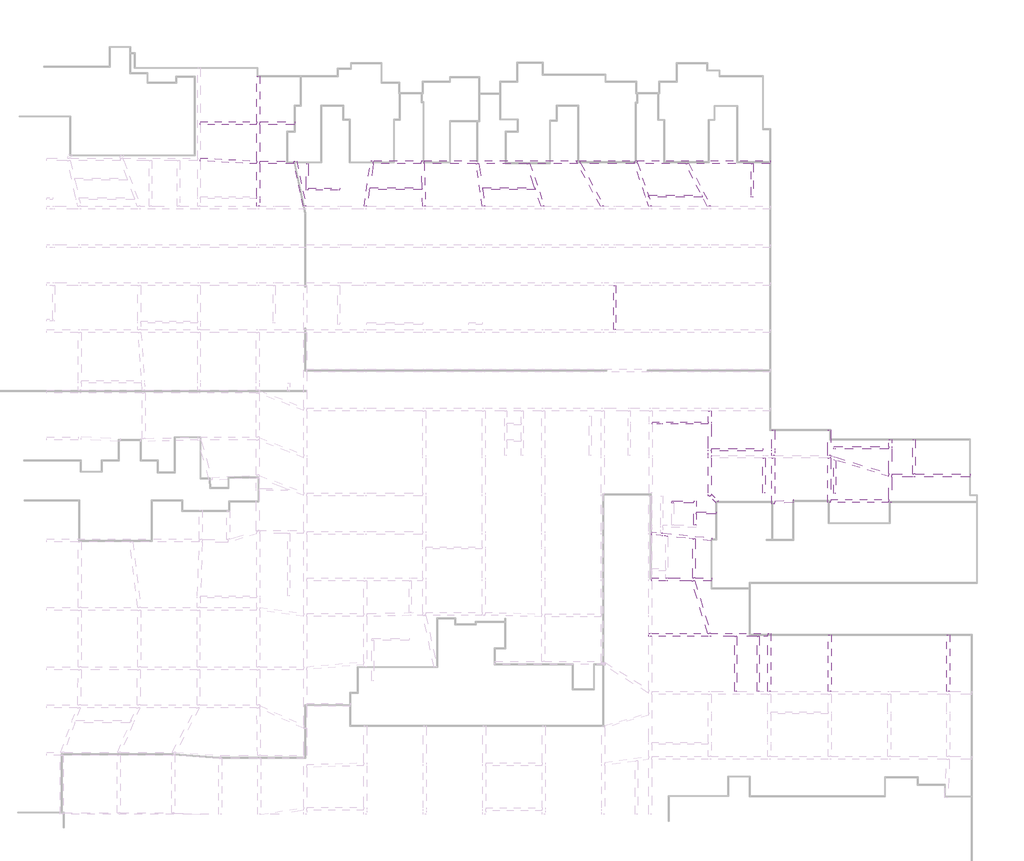
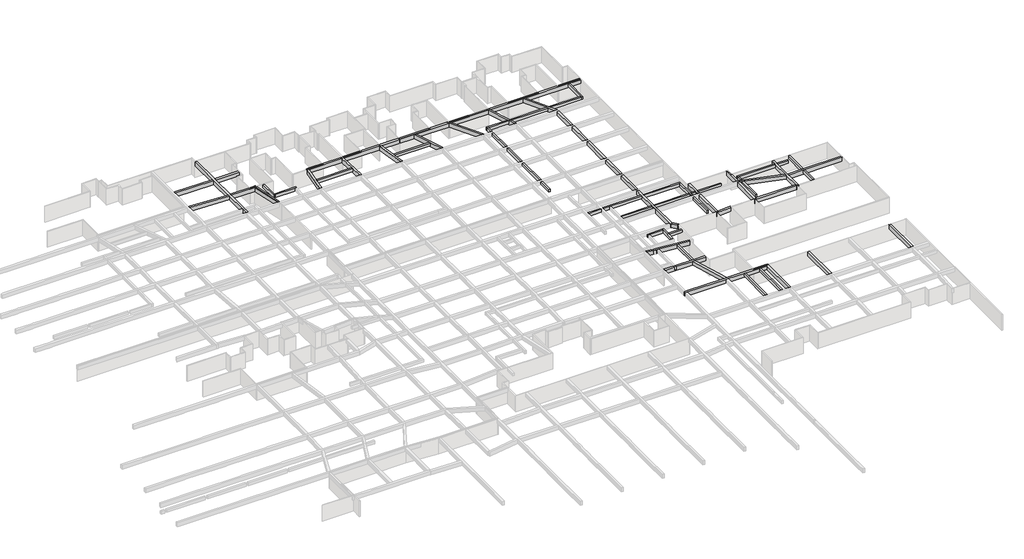
# One storey, part 16 of 16: 54 beams.
"""IFC4 building model written with IfcOpenShell, lengths in millimetres."""

from ifc_helpers import new_model, si_unit, frame, origin, place, context, project, spatial, polyline, outline, extrude, faceted_brep, element, save

model = new_model("IFC4")

# Units and contexts
model_context = context("Model", 3, world=origin())
ifc_project = project(units=[si_unit("LENGTHUNIT", "METRE", prefix="MILLI")], contexts=[model_context])

# Site, building, storey
site = spatial("IfcSite", under=ifc_project)
building = spatial("IfcBuilding", under=site)
storey = spatial("IfcBuildingStorey", under=building, Name="户型图", Elevation=0.0)

# Beams
placement = place(None, origin())
element("IfcBeam", 1, ObjectType="混凝土 - 矩形梁 : KL_beam", at=placement, inside=storey, context=model_context, shape_type="Brep", body=[
    faceted_brep([(134874.2374796, 207962.1094056, 3300.0), (135274.2374796, 207962.1094056, 3300.0), (135274.2374796, 207962.1094056, 2500.0), (134874.2374796, 207962.1094056, 2500.0), (134874.2374796, 201812.9009701, 3300.0), (134874.2374796, 201412.9009701, 3300.0), (134874.2374796, 196462.0408085, 3300.0), (134874.2374796, 196061.4918701, 3300.0), (134874.2374796, 191637.5884701, 3300.0), (134874.2374796, 191337.5884701, 3300.0), (134874.2374796, 190295.7397162, 3300.0), (135274.2374796, 190295.7397162, 3300.0), (135274.2374796, 191337.5884701, 3300.0), (135274.2374796, 191637.5884701, 3300.0), (135274.2374796, 196067.301294, 3300.0), (135274.2374796, 196467.301294, 3300.0), (135274.2374796, 201412.9009701, 3300.0), (135274.2374796, 201812.9009701, 3300.0), (135274.2374796, 190295.7397162, 2500.0), (135274.2374796, 196067.301294, 2500.0), (135274.2374796, 196467.301294, 2500.0), (135274.2374796, 201412.9009701, 2500.0), (135274.2374796, 201812.9009701, 2500.0), (134874.2374796, 190295.7397162, 2500.0), (134874.2374796, 196061.4918701, 2500.0), (134874.2374796, 196462.0408085, 2500.0), (134874.2374796, 201412.9009701, 2500.0), (134874.2374796, 201812.9009701, 2500.0)], [[[0, 1, 2, 3]], [[1, 0, 4, 5, 6, 7, 8, 9, 10, 11, 12, 13, 14, 15, 16, 17]], [[2, 1, 17, 16, 15, 14, 13, 12, 11, 18, 19, 20, 21, 22]], [[3, 2, 22, 21, 20, 19, 18, 23, 24, 25, 26, 27]], [[0, 3, 27, 26, 25, 24, 23, 10, 9, 8, 7, 6, 5, 4]], [[11, 10, 23, 18]]]),
])
element("IfcBeam", 2, ObjectType="混凝土 - 矩形梁 : KL_beam", at=placement, inside=storey, context=model_context, shape_type="SweptSolid", body=[
    extrude(outline(polyline([(127216.2109037, 196462.8320366), (127216.2109037, 196863.380975), (134874.2374796, 196462.0408085), (134874.2374796, 196061.4918701), (127216.2109037, 196462.8320366)])), frame((0.0, 0.0, 2500.0), z_axis=(0.0, 0.0, 1.0), x_axis=(1.0, 0.0, 0.0)), (0.0, 0.0, 1.0), 800.0),
])
element("IfcBeam", 3, ObjectType="混凝土 - 矩形梁 : KL_beam", at=placement, inside=storey, context=model_context, shape_type="SweptSolid", body=[
    extrude(outline(polyline([(127216.2109037, 201412.9009701), (127216.2109037, 201812.9009701), (134874.2374796, 201812.9009701), (134874.2374796, 201412.9009701), (127216.2109037, 201412.9009701)])), frame((0.0, 0.0, 2500.0), z_axis=(0.0, 0.0, 1.0), x_axis=(1.0, 0.0, 0.0)), (0.0, 0.0, 1.0), 800.0),
])
element("IfcBeam", 4, ObjectType="混凝土 - 矩形梁 : KL_beam", at=placement, inside=storey, context=model_context, shape_type="Brep", body=[
    faceted_brep([(196626.5590225, 189895.7397162, 3300.0), (196226.5590225, 189895.7397162, 3300.0), (196226.5590225, 185072.5884701, 3300.0), (196626.5590225, 185072.5884701, 3300.0), (196226.5590225, 189895.7397162, 2500.0), (196226.5590225, 185072.5884701, 2500.0), (196626.5590225, 189895.7397162, 2500.0), (196626.5590225, 185072.5884701, 2500.0)], [[[0, 1, 2, 3]], [[1, 4, 5, 2]], [[4, 6, 7, 5]], [[6, 0, 3, 7]], [[1, 0, 6, 4]], [[3, 2, 5, 7]]]),
    faceted_brep([(196226.5590225, 184672.5884701, 3300.0), (196626.5590225, 184672.5884701, 3300.0), (196626.5590225, 184672.5884701, 2500.0), (196226.5590225, 184672.5884701, 2500.0), (196626.5590225, 179912.5884701, 3300.0), (196226.5590225, 179912.5884701, 3300.0), (196226.5590225, 179912.5884701, 2500.0), (196626.5590225, 179912.5884701, 2500.0)], [[[0, 1, 2, 3]], [[4, 5, 6, 7]], [[1, 0, 5, 4]], [[0, 3, 6, 5]], [[3, 2, 7, 6]], [[2, 1, 4, 7]]]),
    faceted_brep([(196626.5590225, 179512.5884701, 3300.0), (196226.5590225, 179512.5884701, 3300.0), (196226.5590225, 173512.5884701, 3300.0), (196626.5590225, 173512.5884701, 3300.0), (196226.5590225, 179512.5884701, 2500.0), (196226.5590225, 173512.5884701, 2500.0), (196626.5590225, 179512.5884701, 2500.0), (196626.5590225, 173512.5884701, 2500.0)], [[[0, 1, 2, 3]], [[1, 4, 5, 2]], [[4, 6, 7, 5]], [[6, 0, 3, 7]], [[1, 0, 6, 4]], [[3, 2, 5, 7]]]),
    faceted_brep([(196226.5590225, 173112.5884701, 3300.0), (196626.5590225, 173112.5884701, 3300.0), (196626.5590225, 173112.5884701, 2500.0), (196226.5590225, 173112.5884701, 2500.0), (196626.5590225, 168162.578939, 3300.0), (196226.5590225, 168162.578939, 3300.0), (196226.5590225, 168162.578939, 2500.0), (196626.5590225, 168162.578939, 2500.0)], [[[0, 1, 2, 3]], [[4, 5, 6, 7]], [[1, 0, 5, 4]], [[0, 3, 6, 5]], [[3, 2, 7, 6]], [[2, 1, 4, 7]]]),
    faceted_brep([(196226.5590225, 162447.0169772, 3300.0), (196626.5590225, 162447.0169772, 3300.0), (196626.5590225, 162447.0169772, 2500.0), (196226.5590225, 162447.0169772, 2500.0), (196626.5590225, 150902.424794, 3300.0), (196343.71631, 150902.424794, 3300.0), (196226.5590225, 150902.424794, 3300.0), (196226.5590225, 150902.424794, 2500.0), (196343.71631, 150902.424794, 2500.0), (196626.5590225, 150902.424794, 2500.0), (196626.5590225, 151185.2675065, 3300.0), (196626.5590225, 156044.0267812, 3300.0), (196626.5590225, 156444.0267812, 3300.0), (196626.5590225, 157037.5884701, 3300.0), (196626.5590225, 157337.5884701, 3300.0), (196626.5590225, 160683.8998965, 3300.0), (196626.5590225, 160983.8998965, 3300.0), (196226.5590225, 160983.8998965, 3300.0), (196226.5590225, 160683.8998965, 3300.0), (196226.5590225, 157337.5884701, 3300.0), (196226.5590225, 157037.5884701, 3300.0), (196226.5590225, 156444.0267812, 3300.0), (196226.5590225, 156044.0267812, 3300.0), (196226.5590225, 151302.424794, 3300.0), (196226.5590225, 156444.0267812, 2500.0), (196226.5590225, 156044.0267812, 2500.0), (196226.5590225, 151302.424794, 2500.0), (196626.5590225, 156444.0267812, 2500.0), (196626.5590225, 156044.0267812, 2500.0), (196626.5590225, 151185.2675065, 2500.0)], [[[0, 1, 2, 3]], [[4, 5, 6, 7, 8, 9]], [[6, 5, 4, 10, 11, 12, 13, 14, 15, 16, 1, 0, 17, 18, 19, 20, 21, 22, 23]], [[7, 6, 23, 22, 21, 20, 19, 18, 17, 0, 3, 24, 25, 26]], [[9, 8, 7, 26, 25, 24, 3, 2, 27, 28, 29]], [[4, 9, 29, 28, 27, 2, 1, 16, 15, 14, 13, 12, 11, 10]]]),
    faceted_brep([(196626.5590225, 162847.0169772, 3300.0), (196226.5590225, 162847.0169772, 3300.0), (196226.5590225, 162847.0169772, 2500.0), (196626.5590225, 162847.0169772, 2500.0), (196226.5590225, 167762.578939, 3300.0), (196626.5590225, 167762.578939, 3300.0), (196626.5590225, 167762.578939, 2500.0), (196226.5590225, 167762.578939, 2500.0)], [[[0, 1, 2, 3]], [[4, 5, 6, 7]], [[1, 0, 5, 4]], [[2, 1, 4, 7]], [[3, 2, 7, 6]], [[0, 3, 6, 5]]]),
])
element("IfcBeam", 5, ObjectType="混凝土 - 矩形梁 : KL_beam", at=placement, inside=storey, context=model_context, shape_type="Brep", body=[
    faceted_brep([(196099.6244537, 190295.7397162, 3300.0), (196548.907663, 190295.7397162, 3300.0), (195913.7595901, 191537.561337, 3300.0), (195760.3201439, 191837.561337, 3300.0), (193586.5946552, 196087.561337, 3300.0), (193137.311446, 196087.561337, 3300.0), (195311.0369347, 191837.561337, 3300.0), (195464.4763809, 191537.561337, 3300.0), (196548.907663, 190295.7397162, 2500.0), (193586.5946552, 196087.561337, 2500.0), (196099.6244537, 190295.7397162, 2500.0), (193137.311446, 196087.561337, 2500.0)], [[[0, 1, 2, 3, 4, 5, 6, 7]], [[1, 8, 9, 4, 3, 2]], [[8, 10, 11, 9]], [[10, 0, 7, 6, 5, 11]], [[1, 0, 10, 8]], [[5, 4, 9, 11]]]),
])
element("IfcBeam", 6, ObjectType="混凝土 - 矩形梁 : KL_beam", at=placement, inside=storey, context=model_context, shape_type="Brep", body=[
    faceted_brep([(186518.1820909, 196487.561337, 3300.0), (186138.318779, 196362.2462768, 3300.0), (186227.4839698, 196091.9628437, 3300.0), (187630.9903471, 191837.561337, 3300.0), (187729.9588888, 191537.561337, 3300.0), (188139.6298053, 190295.7397162, 3300.0), (188560.8339464, 190295.7397162, 3300.0), (188151.1630299, 191537.561337, 3300.0), (188052.1944881, 191837.561337, 3300.0), (186650.1401466, 196087.561337, 3300.0), (186518.1820909, 196487.561337, 2500.0), (188560.8339464, 190295.7397162, 2500.0), (186650.1401466, 196087.561337, 2500.0), (186138.318779, 196362.2462768, 2500.0), (188139.6298053, 190295.7397162, 2500.0), (186227.4839698, 196091.9628437, 2500.0)], [[[0, 1, 2, 3, 4, 5, 6, 7, 8, 9]], [[10, 0, 9, 8, 7, 6, 11, 12]], [[13, 10, 12, 11, 14, 15]], [[1, 13, 15, 14, 5, 4, 3, 2]], [[6, 5, 14, 11]], [[1, 0, 10, 13]]]),
])
element("IfcBeam", 7, ObjectType="混凝土 - 矩形梁 : KL_beam", at=placement, inside=storey, context=model_context, shape_type="Brep", body=[
    faceted_brep([(178695.0800904, 196491.9628437, 3300.0), (178240.6525334, 196491.9628437, 3300.0), (178456.3013326, 196091.9628437, 3300.0), (181581.1727256, 190295.7397162, 3300.0), (182035.6002826, 190295.7397162, 3300.0), (178910.7288896, 196091.9628437, 3300.0), (178695.0800904, 196491.9628437, 2500.0), (182035.6002826, 190295.7397162, 2500.0), (178910.7288896, 196091.9628437, 2500.0), (178240.6525334, 196491.9628437, 2500.0), (181581.1727256, 190295.7397162, 2500.0), (178456.3013326, 196091.9628437, 2500.0)], [[[0, 1, 2, 3, 4, 5]], [[6, 0, 5, 4, 7, 8]], [[9, 6, 8, 7, 10, 11]], [[1, 9, 11, 10, 3, 2]], [[4, 3, 10, 7]], [[1, 0, 6, 9]]]),
])
element("IfcBeam", 8, ObjectType="混凝土 - 矩形梁 : KL_beam", at=placement, inside=storey, context=model_context, shape_type="Brep", body=[
    faceted_brep([(173535.6280152, 190295.7397162, 3300.0), (173958.7712722, 190295.7397162, 3300.0), (171958.7479668, 196091.9628437, 3300.0), (171535.6047097, 196091.9628437, 3300.0), (172649.8705169, 192862.7338522, 3300.0), (172753.3874068, 192562.7338522, 3300.0), (173958.7712722, 190295.7397162, 2500.0), (171958.7479668, 196091.9628437, 2500.0), (173535.6280152, 190295.7397162, 2500.0), (171535.6047097, 196091.9628437, 2500.0)], [[[0, 1, 2, 3, 4, 5]], [[1, 6, 7, 2]], [[6, 8, 9, 7]], [[8, 0, 5, 4, 3, 9]], [[1, 0, 8, 6]], [[3, 2, 7, 9]]]),
])
element("IfcBeam", 9, ObjectType="混凝土 - 矩形梁 : KL_beam", at=placement, inside=storey, context=model_context, shape_type="Brep", body=[
    faceted_brep([(165485.7043374, 190295.7397162, 3300.0), (165889.741752, 190295.7397162, 3300.0), (165566.8327062, 192562.7338522, 3300.0), (165524.1009178, 192862.7338522, 3300.0), (165064.1318178, 196091.9628437, 3300.0), (164660.0944032, 196091.9628437, 3300.0), (165889.741752, 190295.7397162, 2500.0), (165064.1318178, 196091.9628437, 2500.0), (165485.7043374, 190295.7397162, 2500.0), (164660.0944032, 196091.9628437, 2500.0)], [[[0, 1, 2, 3, 4, 5]], [[1, 6, 7, 4, 3, 2]], [[6, 8, 9, 7]], [[8, 0, 5, 9]], [[1, 0, 8, 6]], [[5, 4, 7, 9]]]),
])
element("IfcBeam", 10, ObjectType="混凝土 - 矩形梁 : KL_beam", at=placement, inside=storey, context=model_context, shape_type="Brep", body=[
    faceted_brep([(157592.9717791, 196491.9628437, 3300.0), (157192.7279613, 196491.9628437, 3300.0), (157206.6962691, 196091.9628437, 3300.0), (157319.4634304, 192862.7338522, 3300.0), (157329.9396612, 192562.7338522, 3300.0), (157409.1048409, 190295.7397162, 3300.0), (157809.3486586, 190295.7397162, 3300.0), (157606.9400869, 196091.9628437, 3300.0), (157592.9717791, 196491.9628437, 2500.0), (157809.3486586, 190295.7397162, 2500.0), (157606.9400869, 196091.9628437, 2500.0), (157192.7279613, 196491.9628437, 2500.0), (157409.1048409, 190295.7397162, 2500.0), (157206.6962691, 196091.9628437, 2500.0)], [[[0, 1, 2, 3, 4, 5, 6, 7]], [[8, 0, 7, 6, 9, 10]], [[11, 8, 10, 9, 12, 13]], [[1, 11, 13, 12, 5, 4, 3, 2]], [[6, 5, 12, 9]], [[1, 0, 8, 11]]]),
])
element("IfcBeam", 11, ObjectType="混凝土 - 矩形梁 : KL_beam", at=placement, inside=storey, context=model_context, shape_type="Brep", body=[
    faceted_brep([(150758.7343587, 196491.9628437, 3300.0), (150354.4344865, 196491.9628437, 3300.0), (149443.4649924, 190295.7397162, 3300.0), (149847.7648646, 190295.7397162, 3300.0), (150181.0586242, 192562.7338522, 3300.0), (150225.1646615, 192862.7338522, 3300.0), (150699.926309, 196091.9628437, 3300.0), (150758.7343587, 196491.9628437, 2500.0), (149847.7648646, 190295.7397162, 2500.0), (150699.926309, 196091.9628437, 2500.0), (150354.4344865, 196491.9628437, 2500.0), (149443.4649924, 190295.7397162, 2500.0)], [[[0, 1, 2, 3, 4, 5, 6]], [[7, 0, 6, 5, 4, 3, 8, 9]], [[10, 7, 9, 8, 11]], [[1, 10, 11, 2]], [[3, 2, 11, 8]], [[1, 0, 7, 10]]]),
])
element("IfcBeam", 12, ObjectType="混凝土 - 矩形梁 : KL_beam", at=placement, inside=storey, context=model_context, shape_type="Brep", body=[
    faceted_brep([(140270.3408026, 196467.301294, 3300.0), (139861.4045646, 196467.301294, 3300.0), (139946.4271893, 196067.301294, 3300.0), (141173.2104737, 190295.7397162, 3300.0), (141582.1467117, 190295.7397162, 3300.0), (140270.3408026, 196467.301294, 2500.0), (141582.1467117, 190295.7397162, 2500.0), (139861.4045646, 196467.301294, 2500.0), (141173.2104737, 190295.7397162, 2500.0), (139946.4271893, 196067.301294, 2500.0)], [[[0, 1, 2, 3, 4]], [[5, 0, 4, 6]], [[7, 5, 6, 8, 9]], [[1, 7, 9, 8, 3, 2]], [[4, 3, 8, 6]], [[1, 0, 5, 7]]]),
])
element("IfcBeam", 13, ObjectType="混凝土 - 矩形梁 : KL_beam", at=placement, inside=storey, context=model_context, shape_type="SweptSolid", body=[
    extrude(outline(polyline([(139861.4045646, 196467.301294), (139946.4271893, 196067.301294), (135274.2374796, 196067.301294), (135274.2374796, 196467.301294), (139861.4045646, 196467.301294)])), frame((0.0, 0.0, 2500.0), z_axis=(0.0, 0.0, 1.0), x_axis=(1.0, 0.0, 0.0)), (0.0, 0.0, 1.0), 800.0),
])
element("IfcBeam", 14, ObjectType="混凝土 - 矩形梁 : KL_beam", at=placement, inside=storey, context=model_context, shape_type="SweptSolid", body=[
    extrude(outline(polyline([(140023.4019686, 201812.9009701), (140023.4019686, 201412.9009701), (135274.2374796, 201412.9009701), (135274.2374796, 201812.9009701), (140023.4019686, 201812.9009701)])), frame((0.0, 0.0, 2500.0), z_axis=(0.0, 0.0, 1.0), x_axis=(1.0, 0.0, 0.0)), (0.0, 0.0, 1.0), 800.0),
])
element("IfcBeam", 15, ObjectType="混凝土 - 矩形梁 : KL_beam", at=placement, inside=storey, context=model_context, shape_type="SweptSolid", body=[
    extrude(outline(polyline([(157192.7279613, 196491.9628437), (157206.6962691, 196091.9628437), (150699.926309, 196091.9628437), (150758.7343587, 196491.9628437), (157192.7279613, 196491.9628437)])), frame((0.0, 0.0, 2500.0), z_axis=(0.0, 0.0, 1.0), x_axis=(1.0, 0.0, 0.0)), (0.0, 0.0, 1.0), 800.0),
])
element("IfcBeam", 16, ObjectType="混凝土 - 矩形梁 : KL_beam", at=placement, inside=storey, context=model_context, shape_type="Brep", body=[
    faceted_brep([(178456.3013326, 196091.9628437, 3300.0), (178240.6525334, 196491.9628437, 3300.0), (157592.9717791, 196491.9628437, 3300.0), (157606.9400869, 196091.9628437, 3300.0), (164660.0944032, 196091.9628437, 3300.0), (165064.1318178, 196091.9628437, 3300.0), (171535.6047097, 196091.9628437, 3300.0), (171958.7479668, 196091.9628437, 3300.0), (178456.3013326, 196091.9628437, 2500.0), (157606.9400869, 196091.9628437, 2500.0), (164660.0944032, 196091.9628437, 2500.0), (165064.1318178, 196091.9628437, 2500.0), (171535.6047097, 196091.9628437, 2500.0), (171958.7479668, 196091.9628437, 2500.0), (178240.6525334, 196491.9628437, 2500.0), (157592.9717791, 196491.9628437, 2500.0)], [[[0, 1, 2, 3, 4, 5, 6, 7]], [[8, 0, 7, 6, 5, 4, 3, 9, 10, 11, 12, 13]], [[14, 8, 13, 12, 11, 10, 9, 15]], [[1, 14, 15, 2]], [[1, 0, 8, 14]], [[3, 2, 15, 9]]]),
])
element("IfcBeam", 17, ObjectType="混凝土 - 矩形梁 : KL_beam", at=placement, inside=storey, context=model_context, shape_type="Brep", body=[
    faceted_brep([(204626.0568509, 196487.561337, 3300.0), (204626.0568509, 196087.561337, 3300.0), (204626.0568509, 196087.561337, 2500.0), (204626.0568509, 196487.561337, 2500.0), (186518.1820909, 196487.561337, 3300.0), (186650.1401466, 196087.561337, 3300.0), (193137.311446, 196087.561337, 3300.0), (193586.5946552, 196087.561337, 3300.0), (202053.5662503, 196087.561337, 3300.0), (202353.5662503, 196087.561337, 3300.0), (186650.1401466, 196087.561337, 2500.0), (193137.311446, 196087.561337, 2500.0), (193586.5946552, 196087.561337, 2500.0), (186518.1820909, 196487.561337, 2500.0)], [[[0, 1, 2, 3]], [[1, 0, 4, 5, 6, 7, 8, 9]], [[2, 1, 9, 8, 7, 6, 5, 10, 11, 12]], [[3, 2, 12, 11, 10, 13]], [[0, 3, 13, 4]], [[5, 4, 13, 10]]]),
])
element("IfcBeam", 18, ObjectType="混凝土 - 矩形梁 : KL_beam", at=placement, inside=storey, context=model_context, shape_type="SweptSolid", body=[
    extrude(outline(polyline([(186516.7300552, 196491.9628437), (186518.1820909, 196487.561337), (186138.318779, 196362.2462768), (186227.4839698, 196091.9628437), (178910.7288896, 196091.9628437), (178695.0800904, 196491.9628437), (186516.7300552, 196491.9628437)])), frame((0.0, 0.0, 2500.0), z_axis=(0.0, 0.0, 1.0), x_axis=(1.0, 0.0, 0.0)), (0.0, 0.0, 1.0), 800.0),
])
element("IfcBeam", 19, ObjectType="混凝土 - 矩形梁 : KL_beam", at=placement, inside=storey, context=model_context, shape_type="Brep", body=[
    faceted_brep([(204846.2265287, 159862.3779382, 3300.0), (205246.2265287, 159862.3779382, 3300.0), (205246.2265287, 159862.3779382, 2500.0), (204846.2265287, 159862.3779382, 2500.0), (204846.2265287, 157337.5884701, 3300.0), (204846.2265287, 157037.5884701, 3300.0), (204846.2265287, 156444.0267812, 3300.0), (205246.2265287, 156444.0267812, 3300.0), (205246.2265287, 157037.5884701, 3300.0), (205246.2265287, 157337.5884701, 3300.0), (205246.2265287, 156444.0267812, 2500.0), (204846.2265287, 156444.0267812, 2500.0)], [[[0, 1, 2, 3]], [[1, 0, 4, 5, 6, 7, 8, 9]], [[2, 1, 9, 8, 7, 10]], [[3, 2, 10, 11]], [[0, 3, 11, 6, 5, 4]], [[7, 6, 11, 10]]]),
])
element("IfcBeam", 20, ObjectType="混凝土 - 矩形梁 : KL_beam", at=placement, inside=storey, context=model_context, shape_type="SweptSolid", body=[
    extrude(outline(polyline([(212466.2091209, 159862.3779382), (212866.2091209, 159862.3779382), (212866.2091209, 156444.0267812), (212466.2091209, 156444.0267812), (212466.2091209, 159862.3779382)])), frame((0.0, 0.0, 2500.0), z_axis=(0.0, 0.0, 1.0), x_axis=(1.0, 0.0, 0.0)), (0.0, 0.0, 1.0), 800.0),
])
element("IfcBeam", 21, ObjectType="混凝土 - 矩形梁 : KL_beam", at=placement, inside=storey, context=model_context, shape_type="SweptSolid", body=[
    extrude(outline(polyline([(228616.2421537, 132011.2586778), (229016.2421537, 132011.2586778), (229016.2421537, 124332.2101355), (228616.2421537, 124332.2101355), (228616.2421537, 132011.2586778)])), frame((0.0, 0.0, 2500.0), z_axis=(0.0, 0.0, 1.0), x_axis=(1.0, 0.0, 0.0)), (0.0, 0.0, 1.0), 800.0),
])
element("IfcBeam", 22, ObjectType="混凝土 - 矩形梁 : KL_beam", at=placement, inside=storey, context=model_context, shape_type="Brep", body=[
    faceted_brep([(204716.2109037, 132211.3072201, 3300.0), (204316.2109037, 132211.3072201, 3300.0), (204316.2109037, 131811.3072201, 3300.0), (204316.2109037, 124332.2101355, 3300.0), (204716.2109037, 124332.2101355, 3300.0), (204716.2109037, 132211.3072201, 2500.0), (204716.2109037, 124332.2101355, 2500.0), (204316.2109037, 132211.3072201, 2500.0), (204316.2109037, 124332.2101355, 2500.0), (204316.2109037, 131811.3072201, 2500.0)], [[[0, 1, 2, 3, 4]], [[5, 0, 4, 6]], [[7, 5, 6, 8, 9]], [[1, 7, 9, 8, 3, 2]], [[4, 3, 8, 6]], [[1, 0, 5, 7]]]),
])
element("IfcBeam", 23, ObjectType="混凝土 - 矩形梁 : KL_beam", at=placement, inside=storey, context=model_context, shape_type="SweptSolid", body=[
    extrude(outline(polyline([(212516.2109037, 132032.2101355), (212916.2109037, 132032.2101355), (212916.2109037, 124332.2101355), (212516.2109037, 124332.2101355), (212516.2109037, 132032.2101355)])), frame((0.0, 0.0, 2500.0), z_axis=(0.0, 0.0, 1.0), x_axis=(1.0, 0.0, 0.0)), (0.0, 0.0, 1.0), 800.0),
])
element("IfcBeam", 24, ObjectType="混凝土 - 矩形梁 : KL_beam", at=placement, inside=storey, context=model_context, shape_type="SweptSolid", body=[
    extrude(outline(polyline([(196576.5767787, 132211.3072201), (196158.3000761, 132211.3072201), (193971.9339862, 139362.5884701), (194390.2106888, 139362.5884701), (196576.5767787, 132211.3072201)])), frame((0.0, 0.0, 2500.0), z_axis=(0.0, 0.0, 1.0), x_axis=(1.0, 0.0, 0.0)), (0.0, 0.0, 1.0), 800.0),
])
element("IfcBeam", 25, ObjectType="混凝土 - 矩形梁 : KL_beam", at=placement, inside=storey, context=model_context, shape_type="Brep", body=[
    faceted_brep([(188116.2109037, 132211.3072201, 3300.0), (188116.2109037, 131811.3072201, 3300.0), (188516.2109037, 131811.3072201, 3300.0), (196255.472134, 131811.3072201, 3300.0), (196655.472134, 131811.3072201, 3300.0), (199816.9298732, 131811.3072201, 3300.0), (200116.9298732, 131811.3072201, 3300.0), (202857.9308744, 131811.3072201, 3300.0), (203157.9308744, 131811.3072201, 3300.0), (204316.2109037, 131811.3072201, 3300.0), (204316.2109037, 132211.3072201, 3300.0), (196576.5767787, 132211.3072201, 3300.0), (196158.3000761, 132211.3072201, 3300.0), (188516.2109037, 132211.3072201, 3300.0), (188116.2109037, 132211.3072201, 2500.0), (204316.2109037, 132211.3072201, 2500.0), (196576.5767787, 132211.3072201, 2500.0), (196158.3000761, 132211.3072201, 2500.0), (188516.2109037, 132211.3072201, 2500.0), (188116.2109037, 131811.3072201, 2500.0), (204316.2109037, 131811.3072201, 2500.0), (196655.472134, 131811.3072201, 2500.0), (196255.472134, 131811.3072201, 2500.0), (188516.2109037, 131811.3072201, 2500.0)], [[[0, 1, 2, 3, 4, 5, 6, 7, 8, 9, 10, 11, 12, 13]], [[14, 0, 13, 12, 11, 10, 15, 16, 17, 18]], [[19, 14, 18, 17, 16, 15, 20, 21, 22, 23]], [[1, 19, 23, 22, 21, 20, 9, 8, 7, 6, 5, 4, 3, 2]], [[10, 9, 20, 15]], [[1, 0, 14, 19]]]),
])
element("IfcBeam", 26, ObjectType="混凝土 - 矩形梁 : KL_beam", at=placement, inside=storey, context=model_context, shape_type="Brep", body=[
    faceted_brep([(196666.2109037, 139762.5884701, 3300.0), (196666.2109037, 139362.5884701, 3300.0), (196666.2109037, 139362.5884701, 2500.0), (196666.2109037, 139762.5884701, 2500.0), (194428.3283765, 139762.5884701, 3300.0), (194128.3283765, 139762.5884701, 3300.0), (190747.6522566, 139762.5884701, 3300.0), (190447.6522566, 139762.5884701, 3300.0), (188516.2109037, 139762.5884701, 3300.0), (188516.2109037, 139362.5884701, 3300.0), (190447.6522566, 139362.5884701, 3300.0), (190747.6522566, 139362.5884701, 3300.0), (193971.9339862, 139362.5884701, 3300.0), (194390.2106888, 139362.5884701, 3300.0), (188516.2109037, 139362.5884701, 2500.0), (193971.9339862, 139362.5884701, 2500.0), (194390.2106888, 139362.5884701, 2500.0), (188516.2109037, 139762.5884701, 2500.0)], [[[0, 1, 2, 3]], [[1, 0, 4, 5, 6, 7, 8, 9, 10, 11, 12, 13]], [[2, 1, 13, 12, 11, 10, 9, 14, 15, 16]], [[3, 2, 16, 15, 14, 17]], [[0, 3, 17, 8, 7, 6, 5, 4]], [[9, 8, 17, 14]]]),
])
element("IfcBeam", 27, ObjectType="混凝土 - 矩形梁 : KL_beam", at=placement, inside=storey, context=model_context, shape_type="Brep", body=[
    faceted_brep([(196686.2077516, 145204.8367157, 3300.0), (196645.3801839, 144806.9257838, 3300.0), (196645.3801839, 144806.9257838, 2500.0), (196686.2077516, 145204.8367157, 2500.0), (190074.1000448, 145883.2706412, 3300.0), (189774.1000448, 145914.0520783, 3300.0), (188516.2109037, 146043.11753, 3300.0), (188516.2109037, 145641.0174941, 3300.0), (189774.1000448, 145511.9520424, 3300.0), (190074.1000448, 145481.1706052, 3300.0), (190447.6522566, 145442.8423588, 3300.0), (190747.6522566, 145412.0609217, 3300.0), (194128.3283765, 145065.187357, 3300.0), (194428.3283765, 145034.4059198, 3300.0), (188516.2109037, 145641.0174941, 2500.0), (188516.2109037, 146043.11753, 2500.0)], [[[0, 1, 2, 3]], [[1, 0, 4, 5, 6, 7, 8, 9, 10, 11, 12, 13]], [[2, 1, 13, 12, 11, 10, 9, 8, 7, 14]], [[3, 2, 14, 15]], [[0, 3, 15, 6, 5, 4]], [[7, 6, 15, 14]]]),
])
element("IfcBeam", 28, ObjectType="混凝土 - 矩形梁 : KL_beam", at=placement, inside=storey, context=model_context, shape_type="SweptSolid", body=[
    extrude(outline(polyline([(197564.4302681, 150247.396261), (197281.5875556, 149964.5535485), (196343.71631, 150902.424794), (196626.5590225, 150902.424794), (196626.5590225, 151185.2675065), (197564.4302681, 150247.396261)])), frame((0.0, 0.0, 2500.0), z_axis=(0.0, 0.0, 1.0), x_axis=(1.0, 0.0, 0.0)), (0.0, 0.0, 1.0), 800.0),
])
element("IfcBeam", 29, ObjectType="混凝土 - 矩形梁 : KL_beam", at=placement, inside=storey, context=model_context, shape_type="Brep", body=[
    faceted_brep([(204846.2265287, 149855.4366597, 3300.0), (205246.2265287, 149855.4366597, 3300.0), (205246.2265287, 150256.126968, 3300.0), (205246.2265287, 156044.0267812, 3300.0), (204846.2265287, 156044.0267812, 3300.0), (204846.2265287, 149855.4366597, 2500.0), (204846.2265287, 156044.0267812, 2500.0), (205246.2265287, 149855.4366597, 2500.0), (205246.2265287, 156044.0267812, 2500.0), (205246.2265287, 150256.126968, 2500.0)], [[[0, 1, 2, 3, 4]], [[5, 0, 4, 6]], [[7, 5, 6, 8, 9]], [[1, 7, 9, 8, 3, 2]], [[4, 3, 8, 6]], [[1, 0, 5, 7]]]),
])
element("IfcBeam", 30, ObjectType="混凝土 - 矩形梁 : KL_beam", at=placement, inside=storey, context=model_context, shape_type="Brep", body=[
    faceted_brep([(207787.1480434, 150405.470045, 3300.0), (207810.6176057, 150006.159164, 3300.0), (207810.6176057, 150006.159164, 2500.0), (207787.1480434, 150405.470045, 2500.0), (205246.2265287, 150256.126968, 3300.0), (205246.2265287, 149855.4366597, 3300.0), (204846.2265287, 149831.9265944, 3300.0), (204846.2265287, 149831.9265944, 2500.0), (205246.2265287, 149855.4366597, 2500.0), (205246.2265287, 150256.126968, 2500.0), (204846.2265287, 149855.4366597, 3300.0), (204846.2265287, 149855.4366597, 2500.0)], [[[0, 1, 2, 3]], [[1, 0, 4, 5]], [[2, 1, 5, 6, 7, 8]], [[3, 2, 8, 9]], [[0, 3, 9, 4]], [[7, 6, 10, 11]], [[8, 5, 4, 9]], [[5, 8, 11, 10]], [[10, 6, 5]], [[8, 7, 11]]]),
])
element("IfcBeam", 31, ObjectType="混凝土 - 矩形梁 : KL_beam", at=placement, inside=storey, context=model_context, shape_type="Brep", body=[
    faceted_brep([(212466.2091209, 150005.8384701, 3300.0), (212866.2091209, 150005.8384701, 3300.0), (212866.2091209, 150405.8384701, 3300.0), (212866.2091209, 155973.7422936, 3300.0), (212866.2091209, 156044.0267812, 3300.0), (212466.2091209, 156044.0267812, 3300.0), (212466.2091209, 150005.8384701, 2500.0), (212466.2091209, 156044.0267812, 2500.0), (212866.2091209, 150005.8384701, 2500.0), (212866.2091209, 156044.0267812, 2500.0), (212866.2091209, 155973.7422936, 2500.0), (212866.2091209, 150405.8384701, 2500.0)], [[[0, 1, 2, 3, 4, 5]], [[6, 0, 5, 7]], [[8, 6, 7, 9, 10, 11]], [[1, 8, 11, 10, 9, 4, 3, 2]], [[5, 4, 9, 7]], [[1, 0, 6, 8]]]),
])
element("IfcBeam", 32, ObjectType="混凝土 - 矩形梁 : KL_beam", at=placement, inside=storey, context=model_context, shape_type="Brep", body=[
    faceted_brep([(212866.2091209, 156392.0189962, 3300.0), (212866.2091209, 156044.0267812, 3300.0), (212866.2091209, 155973.7422936, 3300.0), (213259.0078203, 155853.6516796, 3300.0), (213559.0078203, 155761.9324752, 3300.0), (220759.2888734, 153560.5856421, 3300.0), (220759.2888734, 153978.8623447, 3300.0), (213559.0078203, 156180.2091778, 3300.0), (213259.0078203, 156271.9283822, 3300.0), (212866.2091209, 155973.7422936, 2500.0), (220759.2888734, 153560.5856421, 2500.0), (212866.2091209, 156044.0267812, 2500.0), (212866.2091209, 156392.0189962, 2500.0), (220759.2888734, 153978.8623447, 2500.0)], [[[0, 1, 2, 3, 4, 5, 6, 7, 8]], [[2, 9, 10, 5, 4, 3]], [[9, 11, 12, 13, 10]], [[12, 0, 8, 7, 6, 13]], [[0, 12, 11, 9, 2, 1]], [[6, 5, 10, 13]]]),
])
element("IfcBeam", 33, ObjectType="混凝土 - 矩形梁 : KL_beam", at=placement, inside=storey, context=model_context, shape_type="Brep", body=[
    faceted_brep([(231798.6698135, 153871.1557797, 3300.0), (231798.6698135, 153471.1557797, 3300.0), (231798.6698135, 153471.1557797, 2500.0), (231798.6698135, 153871.1557797, 2500.0), (224324.3359037, 153871.1557797, 3300.0), (224024.3359037, 153871.1557797, 3300.0), (221159.2888734, 153871.1557797, 3300.0), (221159.2888734, 153471.1557797, 3300.0), (224024.3359037, 153471.1557797, 3300.0), (224324.3359037, 153471.1557797, 3300.0), (221159.2888734, 153471.1557797, 2500.0), (221159.2888734, 153871.1557797, 2500.0)], [[[0, 1, 2, 3]], [[1, 0, 4, 5, 6, 7, 8, 9]], [[2, 1, 9, 8, 7, 10]], [[3, 2, 10, 11]], [[0, 3, 11, 6, 5, 4]], [[6, 11, 10, 7]]]),
])
element("IfcBeam", 34, ObjectType="混凝土 - 矩形梁 : KL_beam", at=placement, inside=storey, context=model_context, shape_type="Brep", body=[
    faceted_brep([(221159.2888734, 158611.0728451, 3300.0), (221159.2888734, 158611.0728451, 2500.0), (220759.2888734, 158611.0728451, 2500.0), (220759.2888734, 158611.0728451, 3300.0), (220759.2888734, 157612.7939348, 3300.0), (220759.2888734, 157312.7939348, 3300.0), (220759.2888734, 153978.8623447, 3300.0), (220759.2888734, 153560.5856421, 3300.0), (220759.2888734, 150405.8384701, 3300.0), (220759.2888734, 150005.8384701, 3300.0), (221159.2888734, 150005.8384701, 3300.0), (221159.2888734, 153471.1557797, 3300.0), (221159.2888734, 153871.1557797, 3300.0), (221159.2888734, 157312.7939348, 3300.0), (221159.2888734, 157612.7939348, 3300.0), (220759.2888734, 153978.8623447, 2500.0), (220759.2888734, 153560.5856421, 2500.0), (220759.2888734, 150405.8384701, 2500.0), (220759.2888734, 150005.8384701, 2500.0), (221159.2888734, 153871.1557797, 2500.0), (221159.2888734, 153471.1557797, 2500.0), (221159.2888734, 150005.8384701, 2500.0)], [[[0, 1, 2, 3]], [[0, 3, 4, 5, 6, 7, 8, 9, 10, 11, 12, 13, 14]], [[3, 2, 15, 16, 17, 18, 9, 8, 7, 6, 5, 4]], [[2, 1, 19, 20, 21, 18, 17, 16, 15]], [[1, 0, 14, 13, 12, 11, 10, 21, 20, 19]], [[10, 9, 18, 21]]]),
])
element("IfcBeam", 35, ObjectType="混凝土 - 矩形梁 : KL_beam", at=placement, inside=storey, context=model_context, shape_type="SweptSolid", body=[
    extrude(outline(polyline([(212866.2091209, 150005.8384701), (212866.2091209, 150405.8384701), (220759.2888734, 150405.8384701), (220759.2888734, 150005.8384701), (212866.2091209, 150005.8384701)])), frame((0.0, 0.0, 2500.0), z_axis=(0.0, 0.0, 1.0), x_axis=(1.0, 0.0, 0.0)), (0.0, 0.0, 1.0), 800.0),
])
element("IfcBeam", 36, ObjectType="混凝土 - 矩形梁 : L_beam", at=placement, inside=storey, context=model_context, shape_type="Brep", body=[
    faceted_brep([(141865.5477073, 196122.8753909, 3300.0), (141865.5477073, 196122.8753909, 2700.0), (141565.5477073, 196122.8753909, 2700.0), (141565.5477073, 196122.8753909, 3300.0), (141565.5477073, 192472.8753909, 3300.0), (141865.5477073, 192472.8753909, 3300.0), (141865.5477073, 192772.8753909, 3300.0), (141565.5477073, 192472.8753909, 2700.0), (141865.5477073, 192772.8753909, 2700.0), (141865.5477073, 192472.8753909, 2700.0)], [[[0, 1, 2, 3]], [[0, 3, 4, 5, 6]], [[3, 2, 7, 4]], [[2, 1, 8, 9, 7]], [[1, 0, 6, 5, 9, 8]], [[5, 4, 7, 9]]]),
])
element("IfcBeam", 37, ObjectType="混凝土 - 矩形梁 : L_beam", at=placement, inside=storey, context=model_context, shape_type="Brep", body=[
    faceted_brep([(146146.1090193, 192472.8753909, 3300.0), (146146.1090193, 192772.8753909, 3300.0), (141865.5477073, 192772.8753909, 3300.0), (141865.5477073, 192472.8753909, 3300.0), (145846.1090193, 192472.8753909, 3300.0), (146146.1090193, 192472.8753909, 2700.0), (141865.5477073, 192472.8753909, 2700.0), (145846.1090193, 192472.8753909, 2700.0), (146146.1090193, 192772.8753909, 2700.0), (141865.5477073, 192772.8753909, 2700.0)], [[[0, 1, 2, 3, 4]], [[5, 0, 4, 3, 6, 7]], [[8, 5, 7, 6, 9]], [[1, 8, 9, 2]], [[3, 2, 9, 6]], [[1, 0, 5, 8]]]),
])
element("IfcBeam", 38, ObjectType="混凝土 - 矩形梁 : L_beam", at=placement, inside=storey, context=model_context, shape_type="SweptSolid", body=[
    extrude(outline(polyline([(157319.4634304, 192862.7338522), (157329.9396612, 192562.7338522), (150181.0586242, 192562.7338522), (150225.1646615, 192862.7338522), (157319.4634304, 192862.7338522)])), frame((0.0, 0.0, 2700.0), z_axis=(0.0, 0.0, 1.0), x_axis=(1.0, 0.0, 0.0)), (0.0, 0.0, 1.0), 600.0),
])
element("IfcBeam", 39, ObjectType="混凝土 - 矩形梁 : L_beam", at=placement, inside=storey, context=model_context, shape_type="SweptSolid", body=[
    extrude(outline(polyline([(172649.8705169, 192862.7338522), (172753.3874068, 192562.7338522), (165566.8327062, 192562.7338522), (165524.1009178, 192862.7338522), (172649.8705169, 192862.7338522)])), frame((0.0, 0.0, 2700.0), z_axis=(0.0, 0.0, 1.0), x_axis=(1.0, 0.0, 0.0)), (0.0, 0.0, 1.0), 600.0),
])
element("IfcBeam", 40, ObjectType="混凝土 - 矩形梁 : L_beam", at=placement, inside=storey, context=model_context, shape_type="Brep", body=[
    faceted_brep([(202053.5662503, 191537.561337, 3300.0), (202353.5662503, 191537.561337, 3300.0), (202353.5662503, 196087.561337, 3300.0), (202053.5662503, 196087.561337, 3300.0), (202053.5662503, 191837.561337, 3300.0), (202053.5662503, 191537.561337, 2700.0), (202053.5662503, 196087.561337, 2700.0), (202053.5662503, 191837.561337, 2700.0), (202353.5662503, 191537.561337, 2700.0), (202353.5662503, 196087.561337, 2700.0)], [[[0, 1, 2, 3, 4]], [[5, 0, 4, 3, 6, 7]], [[8, 5, 7, 6, 9]], [[1, 8, 9, 2]], [[3, 2, 9, 6]], [[1, 0, 5, 8]]]),
])
element("IfcBeam", 41, ObjectType="混凝土 - 矩形梁 : L_beam", at=placement, inside=storey, context=model_context, shape_type="Brep", body=[
    faceted_brep([(202053.5662503, 191537.561337, 3300.0), (202053.5662503, 191837.561337, 3300.0), (195760.3201439, 191837.561337, 3300.0), (195913.7595901, 191537.561337, 3300.0), (202053.5662503, 191837.561337, 2700.0), (195760.3201439, 191837.561337, 2700.0), (202053.5662503, 191537.561337, 2700.0), (195913.7595901, 191537.561337, 2700.0)], [[[0, 1, 2, 3]], [[1, 4, 5, 2]], [[4, 6, 7, 5]], [[6, 0, 3, 7]], [[1, 0, 6, 4]], [[3, 2, 5, 7]]]),
    faceted_brep([(195311.0369347, 191837.561337, 3300.0), (195464.4763809, 191537.561337, 3300.0), (195464.4763809, 191537.561337, 2700.0), (195311.0369347, 191837.561337, 2700.0), (188151.1630299, 191537.561337, 3300.0), (188052.1944881, 191837.561337, 3300.0), (188052.1944881, 191837.561337, 2700.0), (188151.1630299, 191537.561337, 2700.0)], [[[0, 1, 2, 3]], [[4, 5, 6, 7]], [[1, 0, 5, 4]], [[0, 3, 6, 5]], [[3, 2, 7, 6]], [[2, 1, 4, 7]]]),
    faceted_brep([(183353.5662503, 191837.561337, 3300.0), (183353.5662503, 191537.561337, 3300.0), (183653.5662503, 191537.561337, 3300.0), (187729.9588888, 191537.561337, 3300.0), (187630.9903471, 191837.561337, 3300.0), (183353.5662503, 191837.561337, 2700.0), (187630.9903471, 191837.561337, 2700.0), (183353.5662503, 191537.561337, 2700.0), (187729.9588888, 191537.561337, 2700.0), (183653.5662503, 191537.561337, 2700.0)], [[[0, 1, 2, 3, 4]], [[5, 0, 4, 6]], [[7, 5, 6, 8, 9]], [[1, 7, 9, 8, 3, 2]], [[4, 3, 8, 6]], [[1, 0, 5, 7]]]),
])
element("IfcBeam", 42, ObjectType="混凝土 - 矩形梁 : L_beam", at=placement, inside=storey, context=model_context, shape_type="SweptSolid", body=[
    extrude(outline(polyline([(183653.5662503, 170334.5470023), (183353.5662503, 170334.5470023), (183353.5662503, 173112.5884701), (183653.5662503, 173112.5884701), (183653.5662503, 170334.5470023)])), frame((0.0, 0.0, 2700.0), z_axis=(0.0, 0.0, 1.0), x_axis=(1.0, 0.0, 0.0)), (0.0, 0.0, 1.0), 600.0),
    extrude(outline(polyline([(183353.5662503, 191537.561337), (183653.5662503, 191537.561337), (183653.5662503, 190295.7397162), (183353.5662503, 190295.7397162), (183353.5662503, 191537.561337)])), frame((0.0, 0.0, 2700.0), z_axis=(0.0, 0.0, 1.0), x_axis=(1.0, 0.0, 0.0)), (0.0, 0.0, 1.0), 600.0),
    extrude(outline(polyline([(183353.5662503, 189895.7397162), (183653.5662503, 189895.7397162), (183653.5662503, 185072.5884701), (183353.5662503, 185072.5884701), (183353.5662503, 189895.7397162)])), frame((0.0, 0.0, 2700.0), z_axis=(0.0, 0.0, 1.0), x_axis=(1.0, 0.0, 0.0)), (0.0, 0.0, 1.0), 600.0),
    extrude(outline(polyline([(183353.5662503, 184672.5884701), (183653.5662503, 184672.5884701), (183653.5662503, 179912.5884701), (183353.5662503, 179912.5884701), (183353.5662503, 184672.5884701)])), frame((0.0, 0.0, 2700.0), z_axis=(0.0, 0.0, 1.0), x_axis=(1.0, 0.0, 0.0)), (0.0, 0.0, 1.0), 600.0),
    extrude(outline(polyline([(183353.5662503, 179512.5884701), (183653.5662503, 179512.5884701), (183653.5662503, 173512.5884701), (183353.5662503, 173512.5884701), (183353.5662503, 179512.5884701)])), frame((0.0, 0.0, 2700.0), z_axis=(0.0, 0.0, 1.0), x_axis=(1.0, 0.0, 0.0)), (0.0, 0.0, 1.0), 600.0),
])
element("IfcBeam", 43, ObjectType="混凝土 - 矩形梁 : L_beam", at=placement, inside=storey, context=model_context, shape_type="Brep", body=[
    faceted_brep([(185653.3391382, 160983.8998965, 3300.0), (185653.3391382, 160683.8998965, 3300.0), (188216.2109037, 160683.8998965, 3300.0), (188216.2109037, 160983.8998965, 3300.0), (185653.3391382, 160683.8998965, 2700.0), (188216.2109037, 160683.8998965, 2700.0), (185653.3391382, 160983.8998965, 2700.0), (188216.2109037, 160983.8998965, 2700.0)], [[[0, 1, 2, 3]], [[1, 4, 5, 2]], [[4, 6, 7, 5]], [[6, 0, 3, 7]], [[1, 0, 6, 4]], [[3, 2, 5, 7]]]),
    faceted_brep([(188616.2109037, 160683.8998965, 3300.0), (188616.2109037, 160983.8998965, 3300.0), (188616.2109037, 160983.8998965, 2700.0), (188616.2109037, 160683.8998965, 2700.0), (196226.5590225, 160983.8998965, 3300.0), (196226.5590225, 160683.8998965, 3300.0), (196226.5590225, 160683.8998965, 2700.0), (196226.5590225, 160983.8998965, 2700.0), (189774.1000448, 160683.8998965, 3300.0), (190074.1000448, 160683.8998965, 3300.0), (189774.1000448, 160683.8998965, 2700.0), (190074.1000448, 160683.8998965, 2700.0)], [[[0, 1, 2, 3]], [[4, 5, 6, 7]], [[1, 0, 8, 9, 5, 4]], [[0, 3, 10, 11, 6, 5, 9, 8]], [[3, 2, 7, 6, 11, 10]], [[2, 1, 4, 7]]]),
    faceted_brep([(203953.3391382, 160683.8998965, 3300.0), (203953.3391382, 160983.8998965, 3300.0), (196626.5590225, 160983.8998965, 3300.0), (196626.5590225, 160683.8998965, 3300.0), (203653.3391382, 160683.8998965, 3300.0), (203953.3391382, 160683.8998965, 2700.0), (196626.5590225, 160683.8998965, 2700.0), (203653.3391382, 160683.8998965, 2700.0), (203953.3391382, 160983.8998965, 2700.0), (196626.5590225, 160983.8998965, 2700.0)], [[[0, 1, 2, 3, 4]], [[5, 0, 4, 3, 6, 7]], [[8, 5, 7, 6, 9]], [[1, 8, 9, 2]], [[3, 2, 9, 6]], [[1, 0, 5, 8]]]),
])
element("IfcBeam", 44, ObjectType="混凝土 - 矩形梁 : L_beam", at=placement, inside=storey, context=model_context, shape_type="Brep", body=[
    faceted_brep([(203953.3391382, 151297.6363531, 3300.0), (203653.3391382, 151297.6363531, 3300.0), (203653.3391382, 151297.6363531, 2700.0), (203953.3391382, 151297.6363531, 2700.0), (203953.3391382, 156044.0267812, 3300.0), (203653.3391382, 156044.0267812, 3300.0), (203653.3391382, 156044.0267812, 2700.0), (203953.3391382, 156044.0267812, 2700.0)], [[[0, 1, 2, 3]], [[1, 0, 4, 5]], [[2, 1, 5, 6]], [[3, 2, 6, 7]], [[0, 3, 7, 4]], [[5, 4, 7, 6]]]),
    faceted_brep([(203653.3391382, 160683.8998965, 3300.0), (203953.3391382, 160683.8998965, 3300.0), (203953.3391382, 160683.8998965, 2700.0), (203653.3391382, 160683.8998965, 2700.0), (203953.3391382, 156444.0267812, 3300.0), (203653.3391382, 156444.0267812, 3300.0), (203653.3391382, 156444.0267812, 2700.0), (203953.3391382, 156444.0267812, 2700.0), (203653.3391382, 157337.5884701, 3300.0), (203653.3391382, 157037.5884701, 3300.0), (203953.3391382, 157037.5884701, 3300.0), (203953.3391382, 157337.5884701, 3300.0), (203653.3391382, 157337.5884701, 2700.0), (203653.3391382, 157037.5884701, 2700.0), (203953.3391382, 157337.5884701, 2700.0), (203953.3391382, 157037.5884701, 2700.0)], [[[0, 1, 2, 3]], [[4, 5, 6, 7]], [[1, 0, 8, 9, 5, 4, 10, 11]], [[0, 3, 12, 13, 6, 5, 9, 8]], [[3, 2, 14, 15, 7, 6, 13, 12]], [[2, 1, 11, 10, 4, 7, 15, 14]]]),
])
element("IfcBeam", 45, ObjectType="混凝土 - 矩形梁 : L_beam", at=placement, inside=storey, context=model_context, shape_type="SweptSolid", body=[
    extrude(outline(polyline([(209830.1060083, 157337.5884701), (209830.1060083, 157037.5884701), (205246.2265287, 157037.5884701), (205246.2265287, 157337.5884701), (209830.1060083, 157337.5884701)])), frame((0.0, 0.0, 2700.0), z_axis=(0.0, 0.0, 1.0), x_axis=(1.0, 0.0, 0.0)), (0.0, 0.0, 1.0), 600.0),
    extrude(outline(polyline([(190074.1000448, 157037.5884701), (190074.1000448, 157337.5884701), (196226.5590225, 157337.5884701), (196226.5590225, 157037.5884701), (190074.1000448, 157037.5884701)])), frame((0.0, 0.0, 2700.0), z_axis=(0.0, 0.0, 1.0), x_axis=(1.0, 0.0, 0.0)), (0.0, 0.0, 1.0), 600.0),
    extrude(outline(polyline([(196626.5590225, 157037.5884701), (196626.5590225, 157337.5884701), (203653.3391382, 157337.5884701), (203653.3391382, 157037.5884701), (196626.5590225, 157037.5884701)])), frame((0.0, 0.0, 2700.0), z_axis=(0.0, 0.0, 1.0), x_axis=(1.0, 0.0, 0.0)), (0.0, 0.0, 1.0), 600.0),
    extrude(outline(polyline([(204846.2265287, 157337.5884701), (204846.2265287, 157037.5884701), (203953.3391382, 157037.5884701), (203953.3391382, 157337.5884701), (204846.2265287, 157337.5884701)])), frame((0.0, 0.0, 2700.0), z_axis=(0.0, 0.0, 1.0), x_axis=(1.0, 0.0, 0.0)), (0.0, 0.0, 1.0), 600.0),
])
element("IfcBeam", 46, ObjectType="混凝土 - 矩形梁 : L_beam", at=placement, inside=storey, context=model_context, shape_type="Brep", body=[
    faceted_brep([(223337.0769083, 157312.7939348, 3300.0), (223337.0769083, 157312.7939348, 2700.0), (223337.0769083, 157612.7939348, 2700.0), (223337.0769083, 157612.7939348, 3300.0), (221159.2888734, 157312.7939348, 3300.0), (221159.2888734, 157612.7939348, 3300.0), (221159.2888734, 157612.7939348, 2700.0), (221159.2888734, 157312.7939348, 2700.0)], [[[0, 1, 2, 3]], [[4, 5, 6, 7]], [[0, 3, 5, 4]], [[3, 2, 6, 5]], [[2, 1, 7, 6]], [[1, 0, 4, 7]]]),
    faceted_brep([(213259.0078203, 157612.7939348, 3300.0), (213259.0078203, 157312.7939348, 3300.0), (213559.0078203, 157312.7939348, 3300.0), (220759.2888734, 157312.7939348, 3300.0), (220759.2888734, 157612.7939348, 3300.0), (213259.0078203, 157612.7939348, 2700.0), (220759.2888734, 157612.7939348, 2700.0), (213259.0078203, 157312.7939348, 2700.0), (220759.2888734, 157312.7939348, 2700.0), (213559.0078203, 157312.7939348, 2700.0)], [[[0, 1, 2, 3, 4]], [[5, 0, 4, 6]], [[7, 5, 6, 8, 9]], [[1, 7, 9, 8, 3, 2]], [[4, 3, 8, 6]], [[1, 0, 5, 7]]]),
])
element("IfcBeam", 47, ObjectType="混凝土 - 矩形梁 : L_beam", at=placement, inside=storey, context=model_context, shape_type="SweptSolid", body=[
    extrude(outline(polyline([(213559.0078203, 151255.7244634), (213259.0078203, 151255.7244634), (213259.0078203, 155853.6516796), (213559.0078203, 155761.9324752), (213559.0078203, 151255.7244634)])), frame((0.0, 0.0, 2700.0), z_axis=(0.0, 0.0, 1.0), x_axis=(1.0, 0.0, 0.0)), (0.0, 0.0, 1.0), 600.0),
    extrude(outline(polyline([(213259.0078203, 157312.7939348), (213559.0078203, 157312.7939348), (213559.0078203, 156180.2091778), (213259.0078203, 156271.9283822), (213259.0078203, 157312.7939348)])), frame((0.0, 0.0, 2700.0), z_axis=(0.0, 0.0, 1.0), x_axis=(1.0, 0.0, 0.0)), (0.0, 0.0, 1.0), 600.0),
])
element("IfcBeam", 48, ObjectType="混凝土 - 矩形梁 : L_beam", at=placement, inside=storey, context=model_context, shape_type="SweptSolid", body=[
    extrude(outline(polyline([(224324.3359037, 150211.3072201), (224024.3359037, 150211.3072201), (224024.3359037, 153471.1557797), (224324.3359037, 153471.1557797), (224324.3359037, 150211.3072201)])), frame((0.0, 0.0, 2700.0), z_axis=(0.0, 0.0, 1.0), x_axis=(1.0, 0.0, 0.0)), (0.0, 0.0, 1.0), 600.0),
    extrude(outline(polyline([(224024.3359037, 158611.3072201), (224324.3359037, 158611.3072201), (224324.3359037, 153871.1557797), (224024.3359037, 153871.1557797), (224024.3359037, 158611.3072201)])), frame((0.0, 0.0, 2700.0), z_axis=(0.0, 0.0, 1.0), x_axis=(1.0, 0.0, 0.0)), (0.0, 0.0, 1.0), 600.0),
])
element("IfcBeam", 49, ObjectType="混凝土 - 矩形梁 : L_beam", at=placement, inside=storey, context=model_context, shape_type="SweptSolid", body=[
    extrude(outline(polyline([(200116.9298732, 124332.2101355), (199816.9298732, 124332.2101355), (199816.9298732, 131811.3072201), (200116.9298732, 131811.3072201), (200116.9298732, 124332.2101355)])), frame((0.0, 0.0, 2700.0), z_axis=(0.0, 0.0, 1.0), x_axis=(1.0, 0.0, 0.0)), (0.0, 0.0, 1.0), 600.0),
])
element("IfcBeam", 50, ObjectType="混凝土 - 矩形梁 : L_beam", at=placement, inside=storey, context=model_context, shape_type="SweptSolid", body=[
    extrude(outline(polyline([(203157.9308744, 124332.2101355), (202857.9308744, 124332.2101355), (202857.9308744, 131811.3072201), (203157.9308744, 131811.3072201), (203157.9308744, 124332.2101355)])), frame((0.0, 0.0, 2700.0), z_axis=(0.0, 0.0, 1.0), x_axis=(1.0, 0.0, 0.0)), (0.0, 0.0, 1.0), 600.0),
])
element("IfcBeam", 51, ObjectType="混凝土 - 矩形梁 : L_beam", at=placement, inside=storey, context=model_context, shape_type="SweptSolid", body=[
    extrude(outline(polyline([(194428.3283765, 139762.5884701), (194128.3283765, 139762.5884701), (194128.3283765, 145065.187357), (194428.3283765, 145034.4059198), (194428.3283765, 139762.5884701)])), frame((0.0, 0.0, 2700.0), z_axis=(0.0, 0.0, 1.0), x_axis=(1.0, 0.0, 0.0)), (0.0, 0.0, 1.0), 600.0),
])
element("IfcBeam", 52, ObjectType="混凝土 - 矩形梁 : L_beam", at=placement, inside=storey, context=model_context, shape_type="Brep", body=[
    faceted_brep([(194566.2109037, 150255.8638084, 3300.0), (194266.2109037, 150255.8638084, 3300.0), (194266.2109037, 149955.8638084, 3300.0), (194266.2109037, 146955.8638084, 3300.0), (194566.2109037, 146955.8638084, 3300.0), (194566.2109037, 148455.8384701, 3300.0), (194566.2109037, 148755.8384701, 3300.0), (194566.2109037, 150255.8638084, 2700.0), (194566.2109037, 146955.8638084, 2700.0), (194566.2109037, 148455.8384701, 2700.0), (194566.2109037, 148755.8384701, 2700.0), (194266.2109037, 150255.8638084, 2700.0), (194266.2109037, 146955.8638084, 2700.0), (194266.2109037, 149955.8638084, 2700.0)], [[[0, 1, 2, 3, 4, 5, 6]], [[7, 0, 6, 5, 4, 8, 9, 10]], [[11, 7, 10, 9, 8, 12, 13]], [[1, 11, 13, 12, 3, 2]], [[4, 3, 12, 8]], [[1, 0, 7, 11]]]),
])
element("IfcBeam", 53, ObjectType="混凝土 - 矩形梁 : L_beam", at=placement, inside=storey, context=model_context, shape_type="Brep", body=[
    faceted_brep([(191266.2109037, 150255.8638084, 3300.0), (191266.2109037, 149955.8638084, 3300.0), (191566.2109037, 149955.8638084, 3300.0), (194266.2109037, 149955.8638084, 3300.0), (194266.2109037, 150255.8638084, 3300.0), (191266.2109037, 150255.8638084, 2700.0), (194266.2109037, 150255.8638084, 2700.0), (191266.2109037, 149955.8638084, 2700.0), (194266.2109037, 149955.8638084, 2700.0), (191566.2109037, 149955.8638084, 2700.0)], [[[0, 1, 2, 3, 4]], [[5, 0, 4, 6]], [[7, 5, 6, 8, 9]], [[1, 7, 9, 8, 3, 2]], [[4, 3, 8, 6]], [[1, 0, 5, 7]]]),
])
element("IfcBeam", 54, ObjectType="混凝土 - 矩形梁 : L_beam", at=placement, inside=storey, context=model_context, shape_type="SweptSolid", body=[
    extrude(outline(polyline([(197316.2109037, 148755.8384701), (197316.2109037, 148455.8384701), (194566.2109037, 148455.8384701), (194566.2109037, 148755.8384701), (197316.2109037, 148755.8384701)])), frame((0.0, 0.0, 2700.0), z_axis=(0.0, 0.0, 1.0), x_axis=(1.0, 0.0, 0.0)), (0.0, 0.0, 1.0), 600.0),
])

save(model, "model.ifc")

# Revit data of these elements
# Type "混凝土 - 矩形梁 : KL_beam"
#   Length [instance default] = 1524 mm
#   b = 400 mm
#   h = 800 mm
#   Structural Material [instance default] = 混凝土 - 现场浇注混凝土
#   Assembly Code = ""
# Type "混凝土 - 矩形梁 : L_beam"
#   Length [instance default] = 1524 mm
#   b = 300 mm
#   h = 600 mm
#   Structural Material [instance default] = none
#   Assembly Code = ""
# Elements 1, 2, 3, 4, 5, 6, 7, 8, 9, 10, 11, 12, 13, 14, 15, 16, 17, 18, 19, 20, 21, 22, 23, 24, 25, 26, 27, 28, 29, 30, 31, 32, 33, 34, 35 (IfcBeam, "混凝土 - 矩形梁 : KL_beam")
#   Comments = ""
#   Structural Material = none
#   Phase Created = 新构造
# Elements 36, 37, 38, 39, 40, 41, 42, 43, 44, 45, 46, 47, 48, 49, 50, 51, 52, 53, 54 (IfcBeam, "混凝土 - 矩形梁 : L_beam")
#   Comments = ""
#   Structural Material = none
#   Phase Created = 新构造
# Materials
#   "混凝土 - 现场浇注混凝土": class "混凝土", colour RGB 192 192 192, transparency 0
